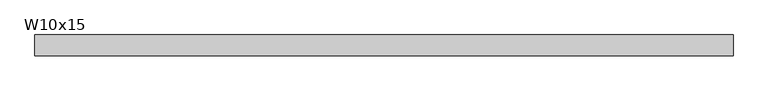
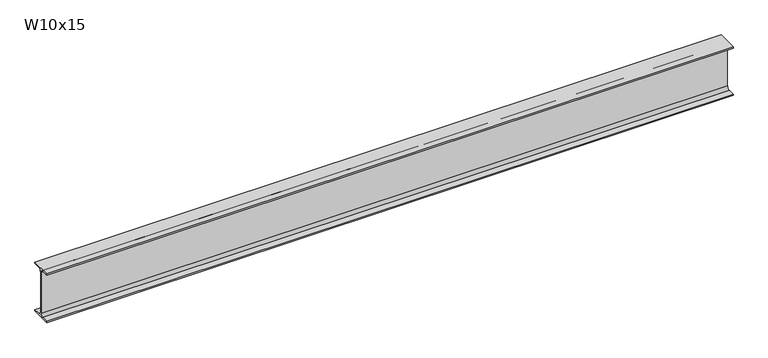
"""IFC4 building model written with IfcOpenShell, lengths in millimetres: beam geometry, RME W-Wide Flange : W10x15."""

from ifc_helpers import new_model, si_unit, point, frame, frame_2d, origin, place, context, project, spatial, polyline, circle_curve, trimmed, segment, composite_curve, outline, extrude, source, transform, mapped, element, save


def w10x15_d4366e7f(model_context):
    return source(origin(), model_context, "Body", "SweptSolid", [
        extrude(outline(composite_curve([segment(polyline([(50.8, -120.142), (50.8, -127.0), (-50.8, -127.0), (-50.8, -120.142), (-16.7005, -120.142)]), True, "CONTINUOUS"), segment(trimmed(circle_curve(frame_2d((-16.7005, -106.3625)), 13.7795), [point((-16.7005, -120.142))], [point((-2.921, -106.3625))], True, "CARTESIAN"), True, "CONTINUOUS"), segment(polyline([(-2.921, -106.3625), (-2.921, 106.3625)]), True, "CONTINUOUS"), segment(trimmed(circle_curve(frame_2d((-16.7005, 106.3625)), 13.7795), [point((-2.921, 106.3625))], [point((-16.7005, 120.142))], True, "CARTESIAN"), True, "CONTINUOUS"), segment(polyline([(-16.7005, 120.142), (-50.8, 120.142), (-50.8, 127.0), (50.8, 127.0), (50.8, 120.142), (16.7005, 120.142)]), True, "CONTINUOUS"), segment(trimmed(circle_curve(frame_2d((16.7005, 106.3625)), 13.7795), [point((16.7005, 120.142))], [point((2.921, 106.3625))], True, "CARTESIAN"), True, "CONTINUOUS"), segment(polyline([(2.921, 106.3625), (2.921, -106.3625)]), True, "CONTINUOUS"), segment(trimmed(circle_curve(frame_2d((16.7005, -106.3625)), 13.7795), [point((2.921, -106.3625))], [point((16.7005, -120.142))], True, "CARTESIAN"), True, "CONTINUOUS"), segment(polyline([(16.7005, -120.142), (50.8, -120.142)]), True, "CONTINUOUS")], self_intersect=False)), frame((-1693.9666248, 0.0, 0.0), z_axis=(1.0, 0.0, 0.0), x_axis=(0.0, 1.0, 0.0)), (0.0, 0.0, 1.0), 3387.9332496),
    ])


if __name__ == "__main__":
    model = new_model("IFC4")
    model_context = context("Model", 3, world=origin())
    ifc_project = project(units=[si_unit("LENGTHUNIT", "METRE", prefix="MILLI")], contexts=[model_context])
    site = spatial("IfcSite", under=ifc_project)
    building = spatial("IfcBuilding", under=site)
    placement = place(None, origin())
    w10x15_shape = w10x15_d4366e7f(model_context)
    element("IfcBeam", 1, ObjectType="RME W-Wide Flange : W10x15", at=placement, inside=building, context=model_context, shape_type="MappedRepresentation", body=[
        mapped(w10x15_shape, transform((0.0, 0.0, 0.0), x_axis=(1.0, 0.0, 0.0), y_axis=(0.0, 1.0, 0.0), z_axis=(0.0, 0.0, 1.0))),
    ])
    save(model, "model.ifc")

# Revit data of these elements
# Type "RME W-Wide Flange : W10x15"
#   WELD P [instance default] = ""
#   WELD LE [instance default] = ""
#   WELD D [instance default] = ""
#   TOP SECTION SIZE [instance default] = ""
#   TOP SECTION LENGTH [instance default] = ""
#   REMARKS [instance default] = ""
#   REINF TYPE [instance default] = ""
#   Nominal Size = "W24"
#   End Bearing Capacity [instance default] = ""
#   BOT SECTION SIZE [instance default] = ""
#   BOT SECTION LENGTH [instance default] = ""
#   Assembly Code = "B10"
#   W = 15
#   Start Extension Calculation [instance default] = 10' - 0"
#   Start Extension [instance default] = -0' - 0 1/2"
#   End Extension Calculation [instance default] = 10' - 0"
#   End Extension [instance default] = -0' - 0 1/2"
#   Length [instance default] = 5' - 0"
#   bf = 0' - 4"
#   d = 0' - 10"
#   k = 0' - 0 13/16"
#   k2 = 0' - 0.5425"
#   tf = 0' - 0.27"
#   tw = 0' - 0.23"
#   A = 0.030625 SF
#   Structural Material [instance default] = Metal - Steel - ASTM A992
# Element 1 (IfcBeam, "RME W-Wide Flange : W10x15")
#   Length = 11' - 1.3832"
#   Materials on its faces: "Metal - Steel - ASTM A992"
# Materials
#   "Metal - Steel - ASTM A992": class "Metal", colour RGB 255 128 0, transparency 0
